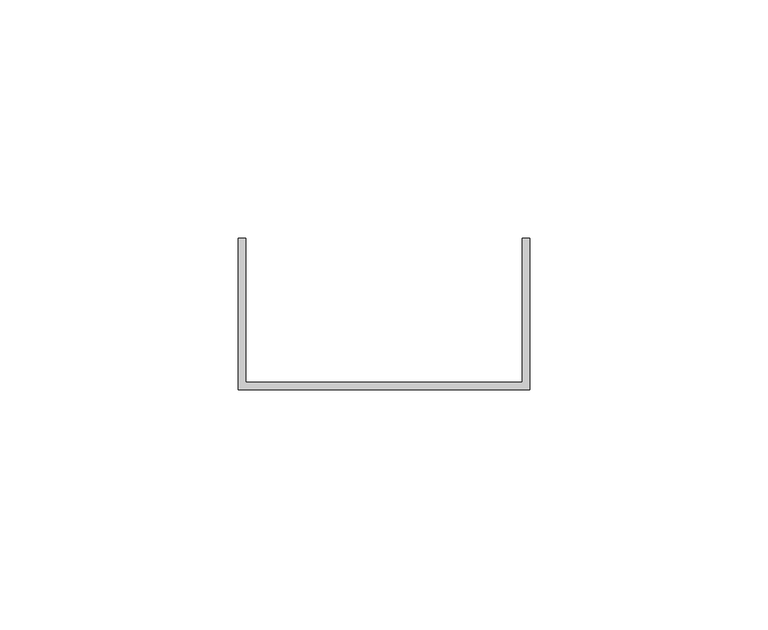
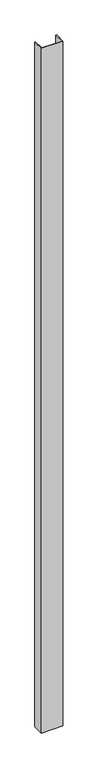
"""IFC4 building model written with IfcOpenShell, lengths in millimetres: proxy geometry, Generic Models 7:Generic Models 1:3:Generic Models 1:3 : Generic Models 7:Generic Models 1:305549:3:Generic Models 1:3:Generic Models 1:3 : Generic Models 7:Generic Models 1:305549:3 : Generic Models 7:Generic Models 1:3:Generic Models 1:3 : Generic Models 7:Generic Models 1:305549:301244:54 : Generic Models 7:Generic Models 1:3:Generic Models 1:3 : Generic Models 7:Generic Models 1:305549:3:Generic Models 1:3:Generic Models 1:3 : Generic Models 7:Generic Models 1:305549:3 : Generic Models 7:Generic Models 1:3:Generic Models 1:3 : Generic Models 7:Generic Models 1:305549:301244:308848."""

from ifc_helpers import new_model, si_unit, frame, origin, place, context, project, spatial, polyline, outline, extrude, source, transform, mapped, element, save


def generic_models_cb70a19b(model_context):
    return source(origin(), model_context, "Body", "SweptSolid", [
        extrude(outline(polyline([(579322.7929739, -578705.4163841), (579322.7929739, -578673.6663841), (579324.3804739, -578673.6663841), (579324.3804739, -578703.8288841), (579382.3242239, -578703.8288841), (579382.3242239, -578673.6663841), (579383.9117239, -578673.6663841), (579383.9117239, -578705.4163841), (579322.7929739, -578705.4163841)])), frame((0.0, 0.0, 4103.2108361), z_axis=(0.0, 0.0, 1.0), x_axis=(1.0, 0.0, 0.0)), (0.0, 0.0, 1.0), 2048.8216016),
    ])


if __name__ == "__main__":
    model = new_model("IFC4")
    model_context = context("Model", 3, world=origin())
    ifc_project = project(units=[si_unit("LENGTHUNIT", "METRE", prefix="MILLI")], contexts=[model_context])
    site = spatial("IfcSite", under=ifc_project)
    building = spatial("IfcBuilding", under=site)
    placement = place(None, origin())
    generic_models_shape = generic_models_cb70a19b(model_context)
    element("IfcBuildingElementProxy", 1, Name="Generic Models 7:Generic Models 1:3:Generic Models 1:3 : Generic Models 7:Generic Models 1:305549:3:Generic Models 1:3:Generic Models 1:3 : Generic Models 7:Generic Models 1:305549:3 : Generic Models 7:Generic Models 1:3:Generic Models 1:3 : Generic Models 7:Generic Models 1:305549:301244:54 : Generic Models 7:Generic Models 1:3:Generic Models 1:3 : Generic Models 7:Generic Models 1:305549:3:Generic Models 1:3:Generic Models 1:3 : Generic Models 7:Generic Models 1:305549:3 : Generic Models 7:Generic Models 1:3:Generic Models 1:3 : Generic Models 7:Generic Models 1:305549:301244:308848", ObjectType="Generic Models 7:Generic Models 1:3:Generic Models 1:3 : Generic Models 7:Generic Models 1:305549:3:Generic Models 1:3:Generic Models 1:3 : Generic Models 7:Generic Models 1:305549:3 : Generic Models 7:Generic Models 1:3:Generic Models 1:3 : Generic Models 7:Generic Models 1:305549:301244:54 : Generic Models 7:Generic Models 1:3:Generic Models 1:3 : Generic Models 7:Generic Models 1:305549:3:Generic Models 1:3:Generic Models 1:3 : Generic Models 7:Generic Models 1:305549:3 : Generic Models 7:Generic Models 1:3:Generic Models 1:3 : Generic Models 7:Generic Models 1:305549:301244:308848", at=placement, inside=building, context=model_context, shape_type="MappedRepresentation", body=[
        mapped(generic_models_shape, transform((0.0, 0.0, 0.0), x_axis=(1.0, 0.0, 0.0), y_axis=(0.0, 1.0, 0.0), z_axis=(0.0, 0.0, 1.0))),
    ])
    save(model, "model.ifc")

# Revit data of these elements
# Type "Generic Models 7:Generic Models 1:3:Generic Models 1:3 : Generic Models 7:Generic Models 1:305549:3:Generic Models 1:3:Generic Models 1:3 : Generic Models 7:Generic Models 1:305549:3 : Generic Models 7:Generic Models 1:3:Generic Models 1:3 : Generic Models 7:Generic Models 1:305549:301244:54 : Generic Models 7:Generic Models 1:3:Generic Models 1:3 : Generic Models 7:Generic Models 1:305549:3:Generic Models 1:3:Generic Models 1:3 : Generic Models 7:Generic Models 1:305549:3 : Generic Models 7:Generic Models 1:3:Generic Models 1:3 : Generic Models 7:Generic Models 1:305549:301244:308848"
#   NameOverride = "Generic Models 7:Generic Models 1:3:Generic Models 1:3 : Generic Models 7:Generic Models 1:305549:3:Generic Models 1:3:Generic Models 1:3 : Generic Models 7:Generic Models 1:305549:3 : Generic Models 7:Generic Models 1:3:Generic Models 1:3 : Generic Models 7:Generic Models 1:305549:301244:308848"
#   ObjectTypeOverride = "Generic Models 1:3:Generic Models 1:3 : Generic Models 7:Generic Models 1:305549:3 : Generic Models 7:Generic Models 1:3:Generic Models 1:3 : Generic Models 7:Generic Models 1:305549:301244"
#   Reference = "Generic Models 1"
#   Tag = "308848"
# Element 1 (IfcBuildingElementProxy, "Generic Models 7:Generic Models 1:3:Generic Models 1:3 : Generic Models 7:Generic Models 1:305549:3:Generic Models 1:3:Generic Models 1:3 : Generic Models 7:Generic Models 1:305549:3 : Generic Models 7:Generic Models 1:3:Generic Models 1:3 : Generic Models 7:Generic Models 1:305549:301244:54 : Generic Models 7:Generic Models 1:3:Generic Models 1:3 : Generic Models 7:Generic Models 1:305549:3:Generic Models 1:3:Generic Models 1:3 : Generic Models 7:Generic Models 1:305549:3 : Generic Models 7:Generic Models 1:3:Generic Models 1:3 : Generic Models 7:Generic Models 1:305549:301244:308848")
#   Materials on its faces: "GALVANIZED U-CHANNEL (250T125-33)"
# Materials
#   "GALVANIZED U-CHANNEL (250T125-33)": class "Unassigned", colour RGB 202 201 200, transparency 0, Keynote = "M05451300.02", Cost = 0
